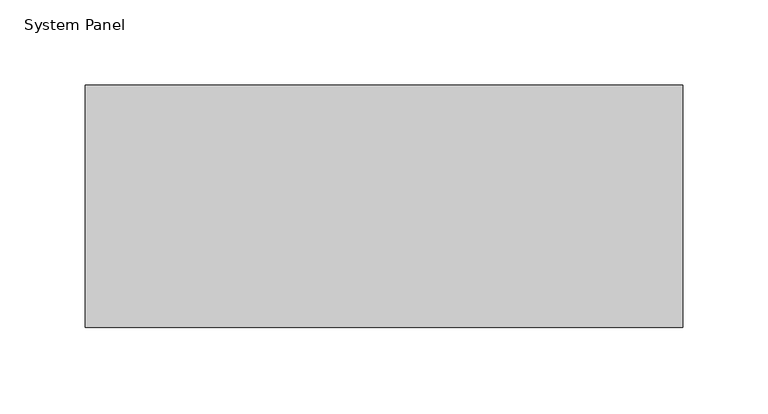
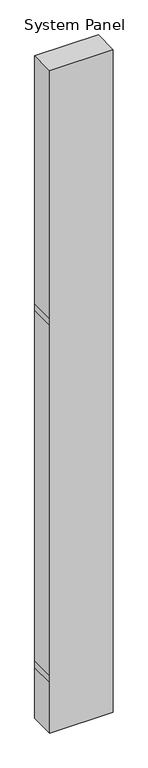
"""IFC4 building model written with IfcOpenShell, lengths in millimetres: plate geometry, System Panel : NLRS_21_CWP_hsb-vulling minerale wol 142 _gen_rsf."""

from ifc_helpers import new_model, si_unit, frame, origin, place, context, project, spatial, polyline, outline, extrude, source, transform, mapped, element, save


def system_panel_360973c8(model_context):
    return source(origin(), model_context, "Body", "SweptSolid", [
        extrude(outline(polyline([(0.0, -175.0000002), (0.0, 175.0000002), (295.0, 175.0000002), (333.0, 175.0000002), (2371.0, 175.0000002), (2409.0, 175.0000002), (3849.0, 175.0000002), (3849.0, -175.0000002), (2409.0, -175.0000002), (2371.0, -175.0000002), (333.0, -175.0000002), (295.0, -175.0000002), (0.0, -175.0000002)])), frame((0.0, -71.0, 0.0), z_axis=(0.0, 1.0, 0.0), x_axis=(0.0, 0.0, 1.0)), (0.0, 0.0, 1.0), 142.0),
    ])


if __name__ == "__main__":
    model = new_model("IFC4")
    model_context = context("Model", 3, world=origin())
    ifc_project = project(units=[si_unit("LENGTHUNIT", "METRE", prefix="MILLI")], contexts=[model_context])
    site = spatial("IfcSite", under=ifc_project)
    building = spatial("IfcBuilding", under=site)
    placement = place(None, origin())
    system_panel_shape = system_panel_360973c8(model_context)
    element("IfcPlate", 1, ObjectType="System Panel : NLRS_21_CWP_hsb-vulling minerale wol 142 _gen_rsf", at=placement, inside=building, context=model_context, shape_type="MappedRepresentation", body=[
        mapped(system_panel_shape, transform((0.0, 0.0, 0.0), x_axis=(1.0, 0.0, 0.0), y_axis=(0.0, 1.0, 0.0), z_axis=(0.0, 0.0, 1.0))),
    ])
    save(model, "model.ifc")

# Revit data of these elements
# Type "System Panel : NLRS_21_CWP_hsb-vulling minerale wol 142 _gen_rsf"
#   Export Type to IFC As = "IfcWall"
#   Type IfcGUID = "07M7mRoiH1CR8m_RSKIwpC"
#   Assembly Code = "21.23"
# Element 1 (IfcPlate, "System Panel : NLRS_21_CWP_hsb-vulling minerale wol 142 _gen_rsf")
#   Materials on its faces: "NLRS_m1_isolatie minerale wol_gen_rsf"
# Materials
#   "NLRS_m1_isolatie minerale wol_gen_rsf": class "M - Anorganische materialen", colour RGB 200 200 140, transparency 0, Keynote = "m1", Manufacturer = "Revit Standards Foundation", URL = "www.revitstandards.org", Description = "isolatie minerale wol", Cost = 0
